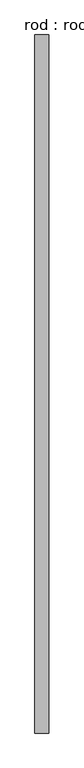
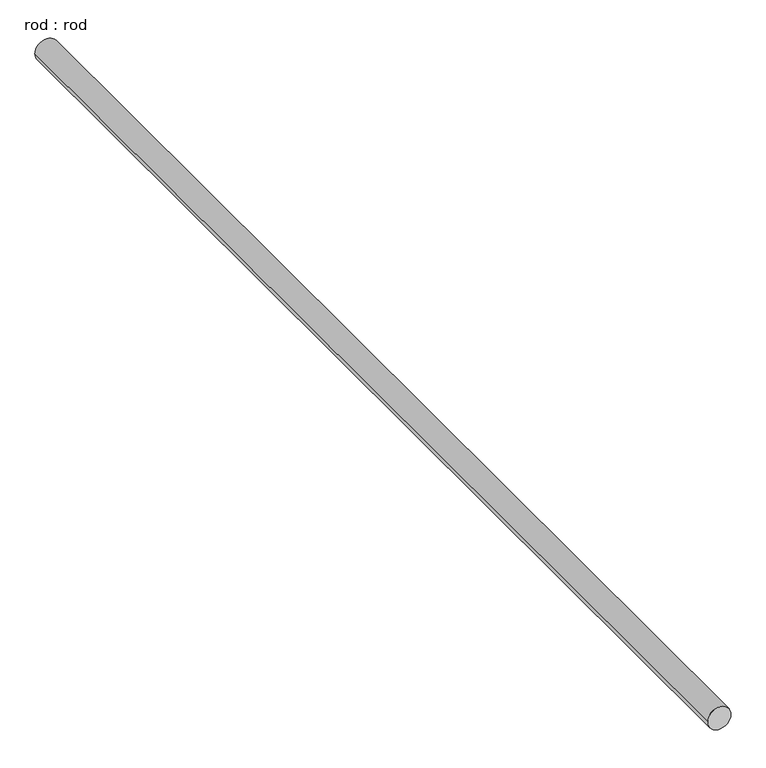
"""IFC4 building model written with IfcOpenShell, lengths in millimetres: proxy geometry, rod : rod."""

from ifc_helpers import new_model, si_unit, point, frame, frame_2d, origin, place, context, project, spatial, circle_curve, trimmed, segment, composite_curve, outline, extrude, source, transform, mapped, element, save


def rod_rod_5aaea62a(model_context):
    return source(origin(), model_context, "Body", "SweptSolid", [
        extrude(outline(composite_curve([segment(trimmed(circle_curve(frame_2d((0.0108462, 0.0)), 200.0), [point((0.0108462, 200.0))], [point((0.0108462, -200.0))], False, "CARTESIAN"), True, "CONTINUOUS"), segment(trimmed(circle_curve(frame_2d((0.0108462, 0.0)), 200.0), [point((0.0108462, -200.0))], [point((0.0108462, 200.0))], False, "CARTESIAN"), True, "CONTINUOUS")], self_intersect=False)), frame((0.0, -5837.4584385, 0.0), z_axis=(0.0, 1.0, 0.0), x_axis=(0.0, 0.0, 1.0)), (0.0, 0.0, 1.0), 19860.3741076),
    ])


if __name__ == "__main__":
    model = new_model("IFC4")
    model_context = context("Model", 3, world=origin())
    ifc_project = project(units=[si_unit("LENGTHUNIT", "METRE", prefix="MILLI")], contexts=[model_context])
    site = spatial("IfcSite", under=ifc_project)
    building = spatial("IfcBuilding", under=site)
    placement = place(None, origin())
    rod_rod_shape = rod_rod_5aaea62a(model_context)
    element("IfcBuildingElementProxy", 1, Name="rod : rod", ObjectType="rod : rod", at=placement, inside=building, context=model_context, shape_type="MappedRepresentation", body=[
        mapped(rod_rod_shape, transform((0.0, 0.0, 0.0), x_axis=(1.0, 0.0, 0.0), y_axis=(0.0, 1.0, 0.0), z_axis=(0.0, 0.0, 1.0))),
    ])
    save(model, "model.ifc")

# Revit data of these elements
# Type "rod : rod"
#   Default Elevation = 0
